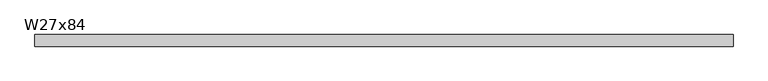
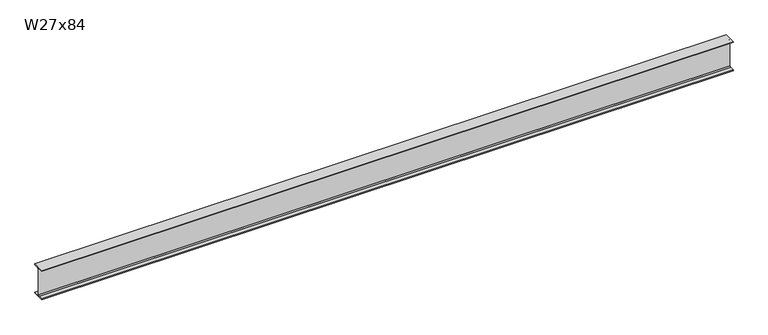
"""IFC4 building model written with IfcOpenShell, lengths in millimetres: beam geometry, RME W-Wide Flange : W27x84."""

from ifc_helpers import new_model, si_unit, point, frame, frame_2d, origin, place, context, project, spatial, polyline, circle_curve, trimmed, segment, composite_curve, outline, extrude, source, transform, mapped, element, save


def w27x84_17ad414c(model_context):
    return source(origin(), model_context, "Body", "SweptSolid", [
        extrude(outline(composite_curve([segment(polyline([(127.0, -322.834), (127.0, -339.09), (-127.0, -339.09), (-127.0, -322.834), (-29.2735, -322.834)]), True, "CONTINUOUS"), segment(trimmed(circle_curve(frame_2d((-29.2735, -299.4025)), 23.4315), [point((-29.2735, -322.834))], [point((-5.842, -299.4025))], True, "CARTESIAN"), True, "CONTINUOUS"), segment(polyline([(-5.842, -299.4025), (-5.842, 299.4025)]), True, "CONTINUOUS"), segment(trimmed(circle_curve(frame_2d((-29.2735, 299.4025)), 23.4315), [point((-5.842, 299.4025))], [point((-29.2735, 322.834))], True, "CARTESIAN"), True, "CONTINUOUS"), segment(polyline([(-29.2735, 322.834), (-127.0, 322.834), (-127.0, 339.09), (127.0, 339.09), (127.0, 322.834), (29.2735, 322.834)]), True, "CONTINUOUS"), segment(trimmed(circle_curve(frame_2d((29.2735, 299.4025)), 23.4315), [point((29.2735, 322.834))], [point((5.842, 299.4025))], True, "CARTESIAN"), True, "CONTINUOUS"), segment(polyline([(5.842, 299.4025), (5.842, -299.4025)]), True, "CONTINUOUS"), segment(trimmed(circle_curve(frame_2d((29.2735, -299.4025)), 23.4315), [point((5.842, -299.4025))], [point((29.2735, -322.834))], True, "CARTESIAN"), True, "CONTINUOUS"), segment(polyline([(29.2735, -322.834), (127.0, -322.834)]), True, "CONTINUOUS")], self_intersect=False)), frame((-7621.9979284, 0.0, 0.0), z_axis=(1.0, 0.0, 0.0), x_axis=(0.0, 1.0, 0.0)), (0.0, 0.0, 1.0), 15251.5841099),
    ])


if __name__ == "__main__":
    model = new_model("IFC4")
    model_context = context("Model", 3, world=origin())
    ifc_project = project(units=[si_unit("LENGTHUNIT", "METRE", prefix="MILLI")], contexts=[model_context])
    site = spatial("IfcSite", under=ifc_project)
    building = spatial("IfcBuilding", under=site)
    placement = place(None, origin())
    w27x84_shape = w27x84_17ad414c(model_context)
    element("IfcBeam", 1, ObjectType="RME W-Wide Flange : W27x84", at=placement, inside=building, context=model_context, shape_type="MappedRepresentation", body=[
        mapped(w27x84_shape, transform((0.0, 0.0, 0.0), x_axis=(1.0, 0.0, 0.0), y_axis=(0.0, 1.0, 0.0), z_axis=(0.0, 0.0, 1.0))),
    ])
    save(model, "model.ifc")

# Revit data of these elements
# Type "RME W-Wide Flange : W27x84"
#   WELD P [instance default] = ""
#   WELD LE [instance default] = ""
#   WELD D [instance default] = ""
#   TOP SECTION SIZE [instance default] = ""
#   TOP SECTION LENGTH [instance default] = ""
#   REMARKS [instance default] = ""
#   REINF TYPE [instance default] = ""
#   Nominal Size = "W24"
#   End Bearing Capacity [instance default] = ""
#   BOT SECTION SIZE [instance default] = ""
#   BOT SECTION LENGTH [instance default] = ""
#   Assembly Code = "B10"
#   W = 84
#   Start Extension Calculation [instance default] = 10' - 0"
#   Start Extension [instance default] = -0' - 0 1/2"
#   End Extension Calculation [instance default] = 10' - 0"
#   End Extension [instance default] = -0' - 0 1/2"
#   Length [instance default] = 5' - 0"
#   bf = 0' - 10"
#   d = 2' - 2.7"
#   k = 0' - 1 9/16"
#   k2 = 0' - 0.9225"
#   tf = 0' - 0.64"
#   tw = 0' - 0.46"
#   A = 0.172222 SF
#   Structural Material [instance default] = Metal - Steel - ASTM A992
# Element 1 (IfcBeam, "RME W-Wide Flange : W27x84")
#   Length = 50' - 10.25303"
#   Materials on its faces: "Metal - Steel - ASTM A992"
# Materials
#   "Metal - Steel - ASTM A992": class "Metal", colour RGB 255 128 0, transparency 0
